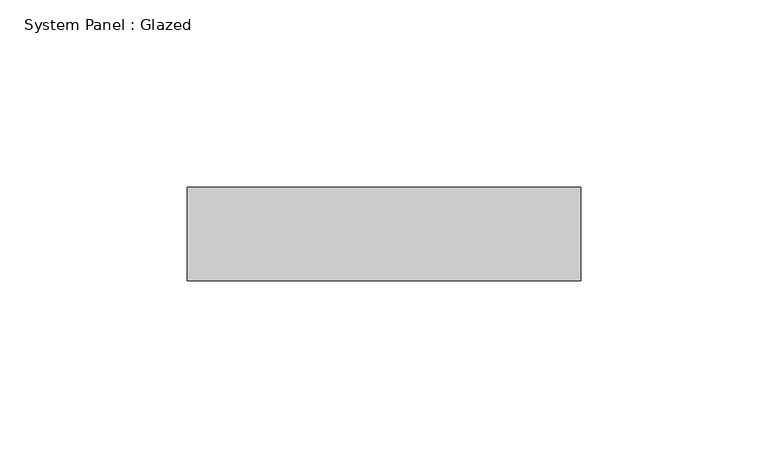
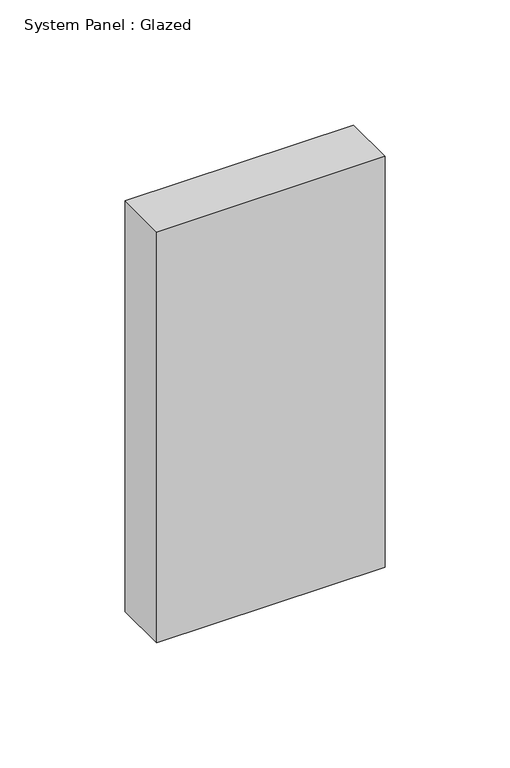
"""IFC4 building model written with IfcOpenShell, lengths in millimetres: plate geometry, System Panel : Glazed."""

from ifc_helpers import new_model, si_unit, origin, origin_with_axes, place, context, project, spatial, polyline, outline, extrude, source, transform, mapped, element, save


def system_panel_glazed_65218e73(model_context):
    return source(origin(), model_context, "Body", "SweptSolid", [
        extrude(outline(polyline([(52.6369119, 24.5), (-52.6369119, 24.5), (-52.6369119, 49.5), (52.6369119, 49.5), (52.6369119, 24.5)])), origin_with_axes(), (0.0, 0.0, 1.0), 200.0),
    ])


if __name__ == "__main__":
    model = new_model("IFC4")
    model_context = context("Model", 3, world=origin())
    ifc_project = project(units=[si_unit("LENGTHUNIT", "METRE", prefix="MILLI")], contexts=[model_context])
    site = spatial("IfcSite", under=ifc_project)
    building = spatial("IfcBuilding", under=site)
    placement = place(None, origin())
    system_panel_glazed_shape = system_panel_glazed_65218e73(model_context)
    element("IfcPlate", 1, ObjectType="System Panel : Glazed", at=placement, inside=building, context=model_context, shape_type="MappedRepresentation", body=[
        mapped(system_panel_glazed_shape, transform((0.0, 0.0, 0.0), x_axis=(1.0, 0.0, 0.0), y_axis=(0.0, 1.0, 0.0), z_axis=(0.0, 0.0, 1.0))),
    ])
    save(model, "model.ifc")

# Revit data of these elements
# Element 1 (IfcPlate, "System Panel : Glazed")
#   Materials on its faces: "Glass"
# Materials
#   "Glass": class "Glass", colour RGB 218 227 224, transparency 0.85, Description = "Soda Lime Glass", Cost = 0
